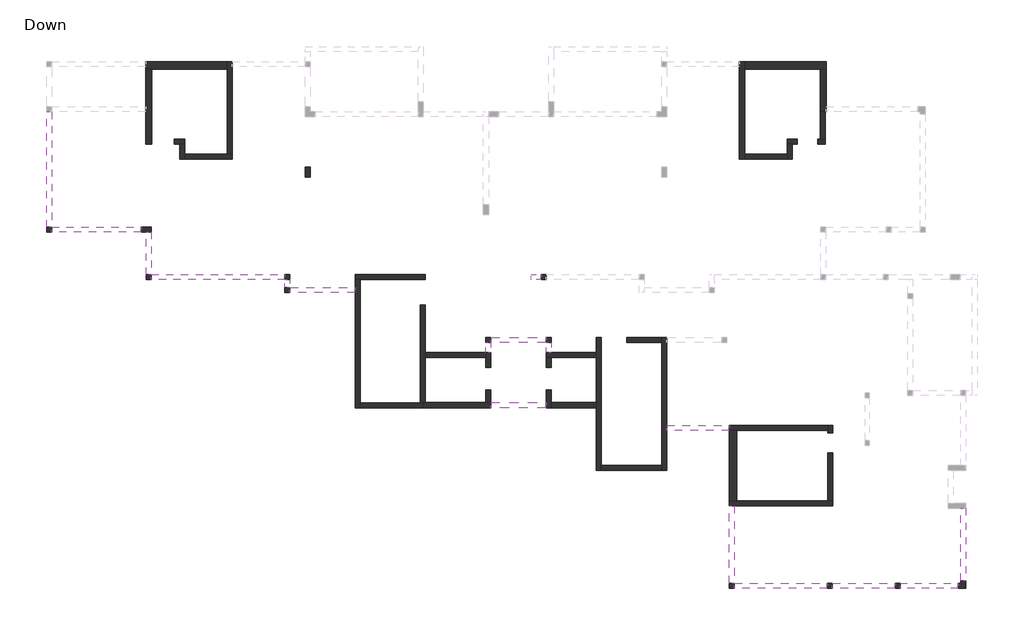
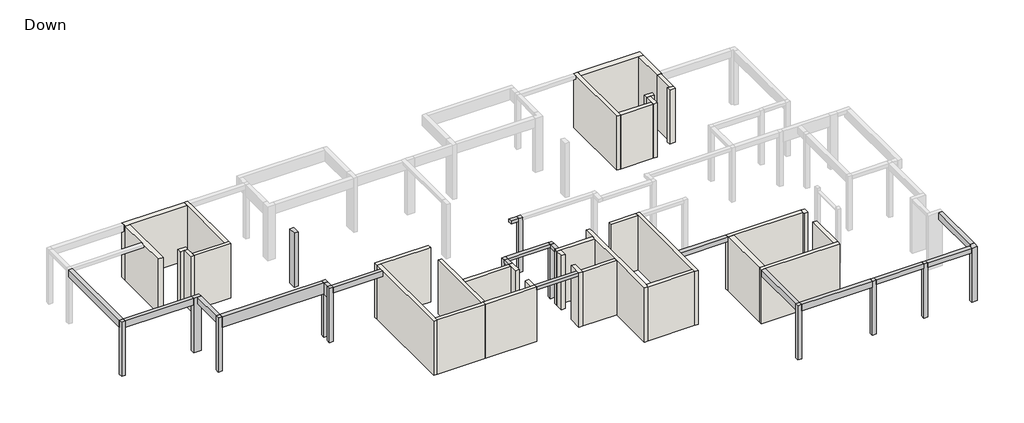
# One storey, part 1 of 2: 35 walls, 17 beams, 13 columns.
"""IFC4 building model written with IfcOpenShell, lengths in millimetres."""

from ifc_helpers import new_model, si_unit, frame, origin, origin_with_axes, place, context, project, spatial, polyline, outline, extrude, faceted_brep, element, save

model = new_model("IFC4")

# Units and contexts
model_context = context("Model", 3, world=origin())
ifc_project = project(units=[si_unit("LENGTHUNIT", "METRE", prefix="MILLI")], contexts=[model_context])

# Site, building, storey
site = spatial("IfcSite", under=ifc_project)
building = spatial("IfcBuilding", under=site)
storey = spatial("IfcBuildingStorey", under=building, Name="Down", Elevation=0.0)

# Beams
placement = place(None, origin())
element("IfcBeam", 1, ObjectType="Concrete Rectengular Beam : 20/15", at=placement, inside=storey, context=model_context, shape_type="SweptSolid", body=[
    extrude(outline(polyline([(23683.1266142, -26322.9713632), (23683.1266142, -26522.9713632), (21465.0782187, -26522.9713632), (21465.0782187, -26322.9713632), (23683.1266142, -26322.9713632)])), frame((0.0, 0.0, 2850.0), z_axis=(0.0, 0.0, 1.0), x_axis=(1.0, 0.0, 0.0)), (0.0, 0.0, 1.0), 150.0),
])
element("IfcBeam", 2, ObjectType="Concrete Rectengular Beam : 20/16", at=placement, inside=storey, context=model_context, shape_type="SweptSolid", body=[
    extrude(outline(polyline([(23683.1266142, -23722.9713632), (23683.1266142, -23922.9713632), (21465.0782187, -23922.9713632), (21465.0782187, -23722.9713632), (23683.1266142, -23722.9713632)])), frame((0.0, 0.0, 2840.0), z_axis=(0.0, 0.0, 1.0), x_axis=(1.0, 0.0, 0.0)), (0.0, 0.0, 1.0), 160.0),
])
element("IfcBeam", 3, ObjectType="Concrete Rectengular Beam : 20/16", at=placement, inside=storey, context=model_context, shape_type="SweptSolid", body=[
    extrude(outline(polyline([(23683.1266142, -23922.9713632), (23883.1266142, -23922.9713632), (23883.1266142, -24325.0312743), (23683.1266142, -24325.0312743), (23683.1266142, -23922.9713632)])), frame((0.0, 0.0, 2840.0), z_axis=(0.0, 0.0, 1.0), x_axis=(1.0, 0.0, 0.0)), (0.0, 0.0, 1.0), 160.0),
])
element("IfcBeam", 4, ObjectType="Concrete Rectengular Beam : 20/16", at=placement, inside=storey, context=model_context, shape_type="SweptSolid", body=[
    extrude(outline(polyline([(21265.0782187, -23922.9713632), (21465.0782187, -23922.9713632), (21465.0782187, -24325.0312743), (21265.0782187, -24325.0312743), (21265.0782187, -23922.9713632)])), frame((0.0, 0.0, 2840.0), z_axis=(0.0, 0.0, 1.0), x_axis=(1.0, 0.0, 0.0)), (0.0, 0.0, 1.0), 160.0),
])
element("IfcBeam", 5, ObjectType="Concrete Rectengular Beam : 20/16", at=placement, inside=storey, context=model_context, shape_type="Brep", body=[
    faceted_brep([(23078.0627315, -21217.3313694, 3000.0), (23078.0627315, -21217.3313694, 2840.0), (23078.0627315, -21325.0312743, 2840.0), (23078.0627315, -21417.3313694, 2840.0), (23078.0627315, -21417.3313694, 3000.0), (23078.0627315, -21325.0312743, 3000.0), (23478.0627315, -21417.3313694, 3000.0), (23478.0627315, -21217.3313694, 3000.0), (23478.0627315, -21217.3313694, 2840.0), (23478.0627315, -21417.3313694, 2840.0)], [[[0, 1, 2, 3, 4, 5]], [[4, 6, 7, 0, 5]], [[1, 0, 7, 8]], [[1, 8, 9, 3, 2]], [[4, 3, 9, 6]], [[7, 6, 9, 8]]]),
])
element("IfcBeam", 6, ObjectType="Concrete Rectengular Beam : 20/25", at=placement, inside=storey, context=model_context, shape_type="SweptSolid", body=[
    extrude(outline(polyline([(37784.3945148, -33727.8618321), (37784.3945148, -33527.8618321), (40096.0050664, -33527.8618321), (40096.0050664, -33727.8618321), (37784.3945148, -33727.8618321)])), frame((0.0, 0.0, 2750.0), z_axis=(0.0, 0.0, 1.0), x_axis=(1.0, 0.0, 0.0)), (0.0, 0.0, 1.0), 250.0),
])
element("IfcBeam", 7, ObjectType="Concrete Rectengular Beam : 20/25", at=placement, inside=storey, context=model_context, shape_type="SweptSolid", body=[
    extrude(outline(polyline([(35086.984967, -33727.8618321), (35086.984967, -33527.8618321), (37584.3945148, -33527.8618321), (37584.3945148, -33727.8618321), (35086.984967, -33727.8618321)])), frame((0.0, 0.0, 2750.0), z_axis=(0.0, 0.0, 1.0), x_axis=(1.0, 0.0, 0.0)), (0.0, 0.0, 1.0), 250.0),
])
element("IfcBeam", 8, ObjectType="Concrete Rectengular Beam : 20/25", at=placement, inside=storey, context=model_context, shape_type="Brep", body=[
    faceted_brep([(30975.7730306, -27429.5129889, 3000.0), (30975.7730306, -27229.5129889, 3000.0), (28484.6380738, -27229.5129889, 3000.0), (28484.6380738, -27429.5129889, 3000.0), (30975.7730306, -27229.5129889, 2840.0), (30975.7730306, -27229.5129889, 2750.0), (28484.6380738, -27229.5129889, 2750.0), (28484.6380738, -27229.5129889, 2840.0), (30975.7730306, -27429.5129889, 2750.0), (28484.6380738, -27429.5129889, 2750.0)], [[[0, 1, 2, 3]], [[2, 1, 4, 5, 6, 7]], [[5, 8, 9, 6]], [[8, 0, 3, 9]], [[1, 0, 8, 5, 4]], [[3, 2, 7, 6, 9]]]),
])
element("IfcBeam", 9, ObjectType="Concrete Rectengular Beam : 20/30", at=placement, inside=storey, context=model_context, shape_type="Brep", body=[
    faceted_brep([(13465.4456872, -21724.9991523, 3000.0), (13465.4456872, -21924.9991523, 3000.0), (16065.0782187, -21924.9991523, 3000.0), (16065.0782187, -21724.9991523, 3000.0), (13465.4456872, -21924.9991523, 2700.0), (16065.0782187, -21924.9991523, 2700.0), (13465.4456872, -21724.9991523, 2700.0), (16065.0782187, -21724.9991523, 2700.0), (16065.0782187, -21724.9991523, 2840.0), (13465.4456872, -21724.9991523, 2840.0)], [[[0, 1, 2, 3]], [[1, 4, 5, 2]], [[4, 6, 7, 5]], [[0, 3, 8, 7, 6, 9]], [[4, 1, 0, 9, 6]], [[3, 2, 5, 7, 8]]]),
])
element("IfcBeam", 10, ObjectType="Concrete Rectengular Beam : 20/35", at=placement, inside=storey, context=model_context, shape_type="Brep", body=[
    faceted_brep([(3964.5925114, -19324.5221497, 3000.0), (3964.5925114, -19524.5221497, 3000.0), (7532.8726521, -19524.5221497, 3000.0), (7532.8726521, -19324.5221497, 3000.0), (3964.5925114, -19524.5221497, 2650.0), (7532.8726521, -19524.5221497, 2650.0), (3964.5925114, -19324.5221497, 2650.0), (7532.8726521, -19324.5221497, 2650.0), (7532.8726521, -19324.5221497, 2840.0), (3964.5925114, -19324.5221497, 2840.0)], [[[0, 1, 2, 3]], [[1, 4, 5, 2]], [[4, 6, 7, 5]], [[0, 3, 8, 7, 6, 9]], [[4, 1, 0, 9, 6]], [[3, 2, 5, 7, 8]]]),
])
element("IfcBeam", 11, ObjectType="Concrete Rectengular Beam : 20/35", at=placement, inside=storey, context=model_context, shape_type="Brep", body=[
    faceted_brep([(7732.8726521, -21217.3313694, 3000.0), (7932.8726521, -21217.3313694, 3000.0), (7932.8726521, -19524.5221497, 3000.0), (7732.8726521, -19524.5221497, 3000.0), (7732.8726521, -21217.3313694, 2650.0), (7732.8726521, -19524.5221497, 2650.0), (7932.8726521, -21217.3313694, 2650.0), (7932.8726521, -19524.5221497, 2650.0), (7932.8726521, -21217.3313694, 2840.0), (7932.8726521, -19524.5221497, 2840.0)], [[[0, 1, 2, 3]], [[4, 0, 3, 5]], [[6, 4, 5, 7]], [[2, 1, 8, 6, 7, 9]], [[3, 2, 9, 7, 5]], [[1, 0, 4, 6, 8]]]),
])
element("IfcBeam", 12, ObjectType="Concrete Rectengular Beam : 20/35", at=placement, inside=storey, context=model_context, shape_type="Brep", body=[
    faceted_brep([(40196.0050664, -33427.8618321, 3000.0), (40396.0050664, -33427.8618321, 3000.0), (40396.0050664, -30530.1793317, 3000.0), (40196.0050664, -30530.1793317, 3000.0), (40196.0050664, -33427.8618321, 2650.0), (40196.0050664, -30530.1793317, 2840.0), (40196.0050664, -30530.1793317, 2650.0), (40396.0050664, -33427.8618321, 2650.0), (40396.0050664, -30530.1793317, 2650.0)], [[[0, 1, 2, 3]], [[4, 0, 3, 5, 6]], [[7, 4, 6, 8]], [[1, 7, 8, 2]], [[1, 0, 4, 7]], [[3, 2, 8, 6, 5]]]),
])
element("IfcBeam", 13, ObjectType="Concrete Rectengular Beam : 20/35", at=placement, inside=storey, context=model_context, shape_type="Brep", body=[
    faceted_brep([(31180.4949796, -33527.8618321, 3000.0), (31180.4949796, -33727.8618321, 3000.0), (34886.984967, -33727.8618321, 3000.0), (34886.984967, -33527.8618321, 3000.0), (31180.4949796, -33527.8618321, 2650.0), (31180.4949796, -33527.8618321, 2840.0), (34886.984967, -33527.8618321, 2650.0), (31180.4949796, -33727.8618321, 2650.0), (34886.984967, -33727.8618321, 2650.0)], [[[0, 1, 2, 3]], [[4, 5, 0, 3, 6]], [[7, 4, 6, 8]], [[1, 7, 8, 2]], [[1, 0, 5, 4, 7]], [[3, 2, 8, 6]]]),
])
element("IfcBeam", 14, ObjectType="Concrete Rectengular Beam : 20/35", at=placement, inside=storey, context=model_context, shape_type="Brep", body=[
    faceted_brep([(30980.4949796, -33527.8618321, 3000.0), (31180.4949796, -33527.8618321, 3000.0), (31180.4949796, -30429.5129889, 3000.0), (30980.4949796, -30429.5129889, 3000.0), (31180.4949796, -33527.8618321, 2840.0), (31180.4949796, -33527.8618321, 2650.0), (31180.4949796, -30429.5129889, 2650.0), (31180.4949796, -30429.5129889, 2840.0), (30980.4949796, -33527.8618321, 2650.0), (30980.4949796, -30429.5129889, 2650.0)], [[[0, 1, 2, 3]], [[1, 4, 5, 6, 7, 2]], [[5, 8, 9, 6]], [[8, 0, 3, 9]], [[0, 8, 5, 4, 1]], [[3, 2, 7, 6, 9]]]),
])
element("IfcBeam", 15, ObjectType="Concrete Rectengular Beam : 20/40", at=placement, inside=storey, context=model_context, shape_type="Brep", body=[
    faceted_brep([(3964.5925114, -14717.2626845, 3000.0), (3764.5925114, -14717.2626845, 3000.0), (3764.5925114, -19324.5221497, 3000.0), (3964.5925114, -19324.5221497, 3000.0), (3764.5925114, -14717.2626845, 2600.0), (3764.5925114, -19324.5221497, 2600.0), (3964.5925114, -14717.2626845, 2600.0), (3964.5925114, -19324.5221497, 2600.0), (3964.5925114, -14717.2626845, 2840.0), (3964.5925114, -19324.5221497, 2840.0)], [[[0, 1, 2, 3]], [[1, 4, 5, 2]], [[4, 6, 7, 5]], [[6, 8, 0, 3, 9, 7]], [[1, 0, 8, 6, 4]], [[3, 2, 5, 7, 9]]]),
])
element("IfcBeam", 16, ObjectType="Concrete Rectengular Beam : 20/60", at=placement, inside=storey, context=model_context, shape_type="Brep", body=[
    faceted_brep([(7932.8726521, -21217.3313694, 3000.0), (7932.8726521, -21417.3313694, 3000.0), (13265.4456872, -21417.3313694, 3000.0), (13265.4456872, -21217.3313694, 3000.0), (7932.8726521, -21417.3313694, 2400.0), (13265.4456872, -21417.3313694, 2400.0), (7932.8726521, -21217.3313694, 2400.0), (13265.4456872, -21217.3313694, 2400.0), (13265.4456872, -21217.3313694, 2840.0), (7932.8726521, -21217.3313694, 2840.0)], [[[0, 1, 2, 3]], [[1, 4, 5, 2]], [[4, 6, 7, 5]], [[0, 3, 8, 7, 6, 9]], [[1, 0, 9, 6, 4]], [[3, 2, 5, 7, 8]]]),
])
element("IfcBeam", 17, ObjectType="Concrete Rectengular Beam : 20/60", at=placement, inside=storey, context=model_context, shape_type="Brep", body=[
    faceted_brep([(13465.4456872, -21417.3313694, 3000.0), (13265.4456872, -21417.3313694, 3000.0), (13265.4456872, -21724.9991523, 3000.0), (13465.4456872, -21724.9991523, 3000.0), (13265.4456872, -21417.3313694, 2400.0), (13265.4456872, -21724.9991523, 2400.0), (13465.4456872, -21417.3313694, 2400.0), (13465.4456872, -21724.9991523, 2400.0), (13465.4456872, -21724.9991523, 2840.0), (13465.4456872, -21417.3313694, 2840.0)], [[[0, 1, 2, 3]], [[1, 4, 5, 2]], [[4, 6, 7, 5]], [[0, 3, 8, 7, 6, 9]], [[4, 1, 0, 9, 6]], [[3, 2, 5, 7, 8]]]),
])

# Columns
element("IfcColumn", 18, ObjectType="Concrete Rectengular Column : 20/20", at=placement, inside=storey, context=model_context, shape_type="SweptSolid", body=[
    extrude(outline(polyline([(31180.4949796, -33527.8618321), (31180.4949796, -33727.8618321), (30980.4949796, -33727.8618321), (30980.4949796, -33527.8618321), (31180.4949796, -33527.8618321)])), origin_with_axes(), (0.0, 0.0, 1.0), 3000.0),
])
element("IfcColumn", 19, ObjectType="Concrete Rectengular Column : 20/20", at=placement, inside=storey, context=model_context, shape_type="SweptSolid", body=[
    extrude(outline(polyline([(35086.984967, -33527.8618321), (35086.984967, -33727.8618321), (34886.984967, -33727.8618321), (34886.984967, -33527.8618321), (35086.984967, -33527.8618321)])), origin_with_axes(), (0.0, 0.0, 1.0), 3000.0),
])
element("IfcColumn", 20, ObjectType="Concrete Rectengular Column : 20/20", at=placement, inside=storey, context=model_context, shape_type="SweptSolid", body=[
    extrude(outline(polyline([(37784.3945148, -33527.8618321), (37784.3945148, -33727.8618321), (37584.3945148, -33727.8618321), (37584.3945148, -33527.8618321), (37784.3945148, -33527.8618321)])), origin_with_axes(), (0.0, 0.0, 1.0), 3000.0),
])
element("IfcColumn", 21, ObjectType="Concrete Rectengular Column : 20/20", at=placement, inside=storey, context=model_context, shape_type="SweptSolid", body=[
    extrude(outline(polyline([(23678.0627315, -21217.3313694), (23678.0627315, -21417.3313694), (23478.0627315, -21417.3313694), (23478.0627315, -21217.3313694), (23678.0627315, -21217.3313694)])), origin_with_axes(), (0.0, 0.0, 1.0), 3000.0),
])
element("IfcColumn", 22, ObjectType="Concrete Rectengular Column : 20/20", at=placement, inside=storey, context=model_context, shape_type="Brep", body=[
    faceted_brep([(23883.1266142, -23722.9713632, 0.0), (23883.1266142, -23922.9713632, 0.0), (23683.1266142, -23922.9713632, 0.0), (23683.1266142, -23722.9713632, 0.0), (23883.1266142, -23722.9713632, 3000.0), (23883.1266142, -23922.9713632, 3000.0), (23883.1266142, -23722.9713632, 2840.0), (23683.1266142, -23922.9713632, 3000.0), (23683.1266142, -23722.9713632, 3000.0)], [[[0, 1, 2, 3]], [[4, 5, 1, 0, 6]], [[5, 7, 2, 1]], [[7, 8, 3, 2]], [[8, 4, 6, 0, 3]], [[4, 8, 7, 5]]]),
])
element("IfcColumn", 23, ObjectType="Concrete Rectengular Column : 20/20", at=placement, inside=storey, context=model_context, shape_type="Brep", body=[
    faceted_brep([(21465.0782187, -23722.9713632, 0.0), (21465.0782187, -23922.9713632, 0.0), (21265.0782187, -23922.9713632, 0.0), (21265.0782187, -23722.9713632, 0.0), (21465.0782187, -23722.9713632, 3000.0), (21465.0782187, -23922.9713632, 3000.0), (21265.0782187, -23922.9713632, 3000.0), (21265.0782187, -23722.9713632, 3000.0), (21265.0782187, -23722.9713632, 2840.0)], [[[0, 1, 2, 3]], [[4, 5, 1, 0]], [[5, 6, 2, 1]], [[6, 7, 8, 3, 2]], [[7, 4, 0, 3, 8]], [[4, 7, 6, 5]]]),
])
element("IfcColumn", 24, ObjectType="Concrete Rectengular Column : 20/20", at=placement, inside=storey, context=model_context, shape_type="SweptSolid", body=[
    extrude(outline(polyline([(3964.5925114, -19324.5221497), (3964.5925114, -19524.5221497), (3764.5925114, -19524.5221497), (3764.5925114, -19324.5221497), (3964.5925114, -19324.5221497)])), origin_with_axes(), (0.0, 0.0, 1.0), 3000.0),
])
element("IfcColumn", 25, ObjectType="Concrete Rectengular Column : 20/20", at=placement, inside=storey, context=model_context, shape_type="SweptSolid", body=[
    extrude(outline(polyline([(7932.8726521, -21217.3313694), (7932.8726521, -21417.3313694), (7732.8726521, -21417.3313694), (7732.8726521, -21217.3313694), (7932.8726521, -21217.3313694)])), origin_with_axes(), (0.0, 0.0, 1.0), 3000.0),
])
element("IfcColumn", 26, ObjectType="Concrete Rectengular Column : 20/20", at=placement, inside=storey, context=model_context, shape_type="Brep", body=[
    faceted_brep([(13465.4456872, -21217.3313694, 0.0), (13465.4456872, -21417.3313694, 0.0), (13265.4456872, -21417.3313694, 0.0), (13265.4456872, -21217.3313694, 0.0), (13465.4456872, -21217.3313694, 3000.0), (13465.4456872, -21417.3313694, 3000.0), (13465.4456872, -21217.3313694, 2840.0), (13265.4456872, -21417.3313694, 3000.0), (13265.4456872, -21217.3313694, 3000.0)], [[[0, 1, 2, 3]], [[4, 5, 1, 0, 6]], [[5, 7, 2, 1]], [[7, 8, 3, 2]], [[8, 4, 6, 0, 3]], [[4, 8, 7, 5]]]),
])
element("IfcColumn", 27, ObjectType="Concrete Rectengular Column : 20/20", at=placement, inside=storey, context=model_context, shape_type="SweptSolid", body=[
    extrude(outline(polyline([(13465.4456872, -21724.9991523), (13465.4456872, -21924.9991523), (13265.4456872, -21924.9991523), (13265.4456872, -21724.9991523), (13465.4456872, -21724.9991523)])), origin_with_axes(), (0.0, 0.0, 1.0), 3000.0),
])
element("IfcColumn", 28, ObjectType="Concrete Rectengular Column : 20/40", at=placement, inside=storey, context=model_context, shape_type="Brep", body=[
    faceted_brep([(7532.8726521, -19324.5221497, 0.0), (7932.8726521, -19324.5221497, 0.0), (7932.8726521, -19524.5221497, 0.0), (7532.8726521, -19524.5221497, 0.0), (7532.8726521, -19324.5221497, 3000.0), (7932.8726521, -19324.5221497, 3000.0), (7932.8726521, -19324.5221497, 2840.0), (7932.8726521, -19524.5221497, 3000.0), (7532.8726521, -19524.5221497, 3000.0)], [[[0, 1, 2, 3]], [[4, 5, 6, 1, 0]], [[5, 7, 2, 1, 6]], [[7, 8, 3, 2]], [[8, 4, 0, 3]], [[4, 8, 7, 5]]]),
])
element("IfcColumn", 29, ObjectType="Concrete Rectengular Column : 20/40", at=placement, inside=storey, context=model_context, shape_type="Brep", body=[
    faceted_brep([(14276.6245949, -16922.7697624, 0.0), (14276.6245949, -17322.7697624, 0.0), (14076.6245949, -17322.7697624, 0.0), (14076.6245949, -16922.7697624, 0.0), (14276.6245949, -16922.7697624, 3000.0), (14276.6245949, -17322.7697624, 3000.0), (14276.6245949, -17322.7697624, 2840.0), (14276.6245949, -16922.7697624, 2840.0), (14076.6245949, -17322.7697624, 3000.0), (14076.6245949, -17322.7697624, 2840.0), (14076.6245949, -16922.7697624, 3000.0), (14076.6245949, -16922.7697624, 2840.0)], [[[0, 1, 2, 3]], [[4, 5, 6, 1, 0, 7]], [[5, 8, 9, 2, 1, 6]], [[8, 10, 11, 3, 2, 9]], [[10, 4, 7, 0, 3, 11]], [[4, 10, 8, 5]]]),
])
element("IfcColumn", 30, ObjectType="L Column : 30/30/20/20", at=placement, inside=storey, context=model_context, shape_type="Brep", body=[
    faceted_brep([(40396.0050664, -33727.8618321, 0.0), (40096.0050664, -33727.8618321, 0.0), (40096.0050664, -33527.8618321, 0.0), (40196.0050664, -33527.8618321, 0.0), (40196.0050664, -33427.8618321, 0.0), (40396.0050664, -33427.8618321, 0.0), (40396.0050664, -33727.8618321, 3000.0), (40096.0050664, -33727.8618321, 3000.0), (40096.0050664, -33527.8618321, 3000.0), (40196.0050664, -33527.8618321, 3000.0), (40196.0050664, -33527.8618321, 2840.0), (40196.0050664, -33427.8618321, 3000.0), (40396.0050664, -33427.8618321, 3000.0)], [[[0, 1, 2, 3, 4, 5]], [[6, 7, 1, 0]], [[7, 8, 2, 1]], [[8, 9, 10, 3, 2]], [[9, 11, 4, 3, 10]], [[11, 12, 5, 4]], [[12, 6, 0, 5]], [[6, 12, 11, 9, 8, 7]]]),
])

# Walls
element("IfcWall", 31, ObjectType="20", at=placement, inside=storey, context=model_context, shape_type="Brep", body=[
    faceted_brep([(8856.7769333, -16016.1045626, 0.0), (9066.7769333, -16016.1045626, 0.0), (9266.7769333, -16016.1045626, 0.0), (9266.7769333, -16016.1045626, 3000.0), (9066.7769333, -16016.1045626, 3000.0), (8856.7769333, -16016.1045626, 3000.0), (8856.7769333, -16016.1045626, 2840.0), (8856.7769333, -15816.1045626, 0.0), (8856.7769333, -15816.1045626, 2840.0), (8856.7769333, -15816.1045626, 3000.0), (9266.7769333, -15816.1045626, 3000.0), (9266.7769333, -15816.1045626, 2840.0), (9266.7769333, -15816.1045626, 0.0)], [[[0, 1, 2, 3, 4, 5, 6]], [[7, 8, 9, 10, 11, 12]], [[2, 1, 0, 7, 12]], [[5, 4, 3, 10, 9]], [[0, 6, 5, 9, 8, 7]], [[3, 2, 12, 11, 10]]]),
])
element("IfcWall", 32, ObjectType="20", at=placement, inside=storey, context=model_context, shape_type="Brep", body=[
    faceted_brep([(9066.7769333, -16016.1045626, 0.0), (9066.7769333, -16605.3286465, 0.0), (9066.7769333, -16605.3286465, 2840.0), (9066.7769333, -16605.3286465, 3000.0), (9066.7769333, -16016.1045626, 3000.0), (9066.7769333, -16016.1045626, 2840.0), (9266.7769333, -16016.1045626, 0.0), (9266.7769333, -16016.1045626, 3000.0), (9266.7769333, -16405.3286465, 3000.0), (9266.7769333, -16605.3286465, 3000.0), (9266.7769333, -16605.3286465, 0.0), (9266.7769333, -16405.3286465, 0.0)], [[[0, 1, 2, 3, 4, 5]], [[6, 7, 8, 9, 10, 11]], [[1, 0, 6, 11, 10]], [[4, 3, 9, 8, 7]], [[0, 5, 4, 7, 6]], [[3, 2, 1, 10, 9]]]),
])
element("IfcWall", 33, ObjectType="20", at=placement, inside=storey, context=model_context, shape_type="Brep", body=[
    faceted_brep([(9266.7769333, -16605.3286465, 0.0), (11166.7769333, -16605.3286465, 0.0), (11166.7769333, -16605.3286465, 2840.0), (11166.7769333, -16605.3286465, 3000.0), (9266.7769333, -16605.3286465, 3000.0), (9266.7769333, -16405.3286465, 0.0), (9266.7769333, -16405.3286465, 2840.0), (9266.7769333, -16405.3286465, 3000.0), (10966.7769333, -16405.3286465, 3000.0), (11166.7769333, -16405.3286465, 3000.0), (11166.7769333, -16405.3286465, 0.0), (10966.7769333, -16405.3286465, 0.0)], [[[0, 1, 2, 3, 4]], [[5, 6, 7, 8, 9, 10, 11]], [[1, 0, 5, 11, 10]], [[4, 3, 9, 8, 7]], [[0, 4, 7, 6, 5]], [[3, 2, 1, 10, 9]]]),
])
element("IfcWall", 34, ObjectType="20", at=placement, inside=storey, context=model_context, shape_type="Brep", body=[
    faceted_brep([(11166.7769333, -16405.3286465, 0.0), (11166.7769333, -12716.1045626, 0.0), (11166.7769333, -12716.1045626, 3000.0), (11166.7769333, -12916.1045626, 3000.0), (11166.7769333, -16405.3286465, 3000.0), (10966.7769333, -16405.3286465, 0.0), (10966.7769333, -16405.3286465, 2840.0), (10966.7769333, -16405.3286465, 3000.0), (10966.7769333, -13016.1045626, 3000.0), (10966.7769333, -12716.1045626, 3000.0), (10966.7769333, -12716.1045626, 0.0), (10966.7769333, -13016.1045626, 0.0)], [[[0, 1, 2, 3, 4]], [[5, 6, 7, 8, 9, 10, 11]], [[1, 0, 5, 11, 10]], [[4, 3, 2, 9, 8, 7]], [[0, 4, 7, 6, 5]], [[2, 1, 10, 9]]]),
])
element("IfcWall", 35, ObjectType="20", at=placement, inside=storey, context=model_context, shape_type="Brep", body=[
    faceted_brep([(35091.7617084, -30229.5129889, 0.0), (34891.7617084, -30229.5129889, 0.0), (31275.7730306, -30229.5129889, 0.0), (30975.7730306, -30229.5129889, 0.0), (30975.7730306, -30229.5129889, 3000.0), (31275.7730306, -30229.5129889, 3000.0), (34891.7617084, -30229.5129889, 3000.0), (35091.7617084, -30229.5129889, 3000.0), (35091.7617084, -30429.5129889, 0.0), (35091.7617084, -30429.5129889, 2840.0), (35091.7617084, -30429.5129889, 3000.0), (31180.4949796, -30429.5129889, 3000.0), (30980.4949796, -30429.5129889, 3000.0), (30975.7730306, -30429.5129889, 3000.0), (30975.7730306, -30429.5129889, 0.0)], [[[0, 1, 2, 3, 4, 5, 6, 7]], [[8, 9, 10, 11, 12, 13, 14]], [[3, 2, 1, 0, 8, 14]], [[7, 6, 5, 4, 13, 12, 11, 10]], [[0, 7, 10, 9, 8]], [[4, 3, 14, 13]]]),
])
element("IfcWall", 36, ObjectType="20", at=placement, inside=storey, context=model_context, shape_type="Brep", body=[
    faceted_brep([(35091.7617084, -30229.5129889, 0.0), (35091.7617084, -28329.5129889, 0.0), (35091.7617084, -28329.5129889, 2840.0), (35091.7617084, -28329.5129889, 3000.0), (35091.7617084, -30229.5129889, 3000.0), (34891.7617084, -30229.5129889, 0.0), (34891.7617084, -30229.5129889, 2840.0), (34891.7617084, -30229.5129889, 3000.0), (34891.7617084, -28329.5129889, 3000.0), (34891.7617084, -28329.5129889, 2840.0), (34891.7617084, -28329.5129889, 0.0)], [[[0, 1, 2, 3, 4]], [[5, 6, 7, 8, 9, 10]], [[1, 0, 5, 10]], [[3, 2, 1, 10, 9, 8]], [[4, 3, 8, 7]], [[0, 4, 7, 6, 5]]]),
])
element("IfcWall", 37, ObjectType="20", at=placement, inside=storey, context=model_context, shape_type="Brep", body=[
    faceted_brep([(35091.7617084, -27529.5129889, 0.0), (35091.7617084, -27229.5129889, 0.0), (35091.7617084, -27229.5129889, 2840.0), (35091.7617084, -27229.5129889, 3000.0), (35091.7617084, -27529.5129889, 3000.0), (35091.7617084, -27529.5129889, 2840.0), (34891.7617084, -27529.5129889, 0.0), (34891.7617084, -27529.5129889, 2840.0), (34891.7617084, -27529.5129889, 3000.0), (34891.7617084, -27429.5129889, 3000.0), (34891.7617084, -27229.5129889, 3000.0), (34891.7617084, -27229.5129889, 0.0), (34891.7617084, -27429.5129889, 0.0)], [[[0, 1, 2, 3, 4, 5]], [[6, 7, 8, 9, 10, 11, 12]], [[1, 0, 6, 12, 11]], [[4, 3, 10, 9, 8]], [[0, 5, 4, 8, 7, 6]], [[3, 2, 1, 11, 10]]]),
])
element("IfcWall", 38, ObjectType="20", at=placement, inside=storey, context=model_context, shape_type="Brep", body=[
    faceted_brep([(34891.7617084, -27229.5129889, 0.0), (30975.7730306, -27229.5129889, 0.0), (30975.7730306, -27229.5129889, 2750.0), (30975.7730306, -27229.5129889, 3000.0), (34891.7617084, -27229.5129889, 3000.0), (34891.7617084, -27429.5129889, 0.0), (34891.7617084, -27429.5129889, 2840.0), (34891.7617084, -27429.5129889, 3000.0), (31275.7730306, -27429.5129889, 3000.0), (30975.7730306, -27429.5129889, 3000.0), (30975.7730306, -27429.5129889, 2750.0), (30975.7730306, -27429.5129889, 0.0), (31275.7730306, -27429.5129889, 0.0)], [[[0, 1, 2, 3, 4]], [[5, 6, 7, 8, 9, 10, 11, 12]], [[1, 0, 5, 12, 11]], [[4, 3, 9, 8, 7]], [[0, 4, 7, 6, 5]], [[3, 2, 1, 11, 10, 9]]]),
])
element("IfcWall", 39, ObjectType="20", at=placement, inside=storey, context=model_context, shape_type="Brep", body=[
    faceted_brep([(28484.6380738, -29030.0312743, 0.0), (28484.6380738, -23722.9713632, 0.0), (28484.6380738, -23722.9713632, 3000.0), (28484.6380738, -23922.9713632, 3000.0), (28484.6380738, -27229.5129889, 3000.0), (28484.6380738, -29030.0312743, 3000.0), (28284.6380738, -29030.0312743, 0.0), (28284.6380738, -29030.0312743, 3000.0), (28284.6380738, -28830.0312743, 3000.0), (28284.6380738, -23922.9713632, 3000.0), (28284.6380738, -23722.9713632, 3000.0), (28284.6380738, -23722.9713632, 0.0), (28284.6380738, -23922.9713632, 0.0), (28284.6380738, -28830.0312743, 0.0)], [[[0, 1, 2, 3, 4, 5]], [[6, 7, 8, 9, 10, 11, 12, 13]], [[1, 0, 6, 13, 12, 11]], [[5, 4, 3, 2, 10, 9, 8, 7]], [[2, 1, 11, 10]], [[0, 5, 7, 6]]]),
])
element("IfcWall", 40, ObjectType="20", at=placement, inside=storey, context=model_context, shape_type="Brep", body=[
    faceted_brep([(28284.6380738, -23722.9713632, 0.0), (26884.6380738, -23722.9713632, 0.0), (26884.6380738, -23722.9713632, 2840.0), (26884.6380738, -23722.9713632, 3000.0), (28284.6380738, -23722.9713632, 3000.0), (28284.6380738, -23922.9713632, 0.0), (28284.6380738, -23922.9713632, 3000.0), (26884.6380738, -23922.9713632, 3000.0), (26884.6380738, -23922.9713632, 2840.0), (26884.6380738, -23922.9713632, 0.0)], [[[0, 1, 2, 3, 4]], [[5, 6, 7, 8, 9]], [[1, 0, 5, 9]], [[3, 2, 1, 9, 8, 7]], [[4, 3, 7, 6]], [[0, 4, 6, 5]]]),
])
element("IfcWall", 41, ObjectType="20", at=placement, inside=storey, context=model_context, shape_type="Brep", body=[
    faceted_brep([(25666.8915333, -23725.0312743, 0.0), (25666.8915333, -24325.0312743, 0.0), (25666.8915333, -24525.0312743, 0.0), (25666.8915333, -26322.9713632, 0.0), (25666.8915333, -26522.9713632, 0.0), (25666.8915333, -29030.0312743, 0.0), (25666.8915333, -29030.0312743, 3000.0), (25666.8915333, -26522.9713632, 3000.0), (25666.8915333, -26322.9713632, 3000.0), (25666.8915333, -24525.0312743, 3000.0), (25666.8915333, -24325.0312743, 3000.0), (25666.8915333, -23725.0312743, 3000.0), (25666.8915333, -23725.0312743, 2840.0), (25866.8915333, -23725.0312743, 0.0), (25866.8915333, -23725.0312743, 2840.0), (25866.8915333, -23725.0312743, 3000.0), (25866.8915333, -23922.9713632, 3000.0), (25866.8915333, -28830.0312743, 3000.0), (25866.8915333, -29030.0312743, 3000.0), (25866.8915333, -29030.0312743, 0.0), (25866.8915333, -28830.0312743, 0.0)], [[[0, 1, 2, 3, 4, 5, 6, 7, 8, 9, 10, 11, 12]], [[13, 14, 15, 16, 17, 18, 19, 20]], [[5, 4, 3, 2, 1, 0, 13, 20, 19]], [[11, 10, 9, 8, 7, 6, 18, 17, 16, 15]], [[0, 12, 11, 15, 14, 13]], [[6, 5, 19, 18]]]),
])
element("IfcWall", 42, ObjectType="20", at=placement, inside=storey, context=model_context, shape_type="SweptSolid", body=[
    extrude(outline(polyline([(28284.6380738, -29030.0312743), (25866.8915333, -29030.0312743), (25866.8915333, -28830.0312743), (28284.6380738, -28830.0312743), (28284.6380738, -29030.0312743)])), origin_with_axes(), (0.0, 0.0, 1.0), 3000.0),
])
element("IfcWall", 43, ObjectType="20", at=placement, inside=storey, context=model_context, shape_type="Brep", body=[
    faceted_brep([(25666.8915333, -24325.0312743, 0.0), (23683.1266142, -24325.0312743, 0.0), (23683.1266142, -24325.0312743, 3000.0), (23883.1266142, -24325.0312743, 3000.0), (25666.8915333, -24325.0312743, 3000.0), (25666.8915333, -24325.0312743, 2840.0), (25666.8915333, -24525.0312743, 0.0), (25666.8915333, -24525.0312743, 3000.0), (23883.1266142, -24525.0312743, 3000.0), (23683.1266142, -24525.0312743, 3000.0), (23683.1266142, -24525.0312743, 0.0), (23883.1266142, -24525.0312743, 0.0)], [[[0, 1, 2, 3, 4, 5]], [[6, 7, 8, 9, 10, 11]], [[1, 0, 6, 11, 10]], [[4, 3, 2, 9, 8, 7]], [[0, 5, 4, 7, 6]], [[2, 1, 10, 9]]]),
])
element("IfcWall", 44, ObjectType="20", at=placement, inside=storey, context=model_context, shape_type="Brep", body=[
    faceted_brep([(23683.1266142, -24525.0312743, 0.0), (23683.1266142, -24925.0312743, 0.0), (23683.1266142, -24925.0312743, 2840.0), (23683.1266142, -24925.0312743, 3000.0), (23683.1266142, -24525.0312743, 3000.0), (23883.1266142, -24525.0312743, 0.0), (23883.1266142, -24525.0312743, 3000.0), (23883.1266142, -24925.0312743, 3000.0), (23883.1266142, -24925.0312743, 2840.0), (23883.1266142, -24925.0312743, 0.0)], [[[0, 1, 2, 3, 4]], [[5, 6, 7, 8, 9]], [[1, 0, 5, 9]], [[3, 2, 1, 9, 8, 7]], [[4, 3, 7, 6]], [[0, 4, 6, 5]]]),
])
element("IfcWall", 45, ObjectType="20", at=placement, inside=storey, context=model_context, shape_type="Brep", body=[
    faceted_brep([(23683.1266142, -25822.9713632, 0.0), (23683.1266142, -26522.9713632, 0.0), (23683.1266142, -26522.9713632, 3000.0), (23683.1266142, -26322.9713632, 3000.0), (23683.1266142, -25822.9713632, 3000.0), (23683.1266142, -25822.9713632, 2840.0), (23883.1266142, -25822.9713632, 0.0), (23883.1266142, -25822.9713632, 2840.0), (23883.1266142, -25822.9713632, 3000.0), (23883.1266142, -26322.9713632, 3000.0), (23883.1266142, -26522.9713632, 3000.0), (23883.1266142, -26522.9713632, 0.0), (23883.1266142, -26322.9713632, 0.0)], [[[0, 1, 2, 3, 4, 5]], [[6, 7, 8, 9, 10, 11, 12]], [[1, 0, 6, 12, 11]], [[4, 3, 2, 10, 9, 8]], [[0, 5, 4, 8, 7, 6]], [[2, 1, 11, 10]]]),
])
element("IfcWall", 46, ObjectType="20", at=placement, inside=storey, context=model_context, shape_type="SweptSolid", body=[
    extrude(outline(polyline([(25666.8915333, -26522.9713632), (23883.1266142, -26522.9713632), (23883.1266142, -26322.9713632), (25666.8915333, -26322.9713632), (25666.8915333, -26522.9713632)])), origin_with_axes(), (0.0, 0.0, 1.0), 3000.0),
])
element("IfcWall", 47, ObjectType="20", at=placement, inside=storey, context=model_context, shape_type="Brep", body=[
    faceted_brep([(21465.0782187, -24925.0312743, 0.0), (21465.0782187, -24325.0312743, 0.0), (21465.0782187, -24325.0312743, 2840.0), (21465.0782187, -24325.0312743, 3000.0), (21465.0782187, -24925.0312743, 3000.0), (21465.0782187, -24925.0312743, 2840.0), (21265.0782187, -24925.0312743, 0.0), (21265.0782187, -24925.0312743, 2840.0), (21265.0782187, -24925.0312743, 3000.0), (21265.0782187, -24525.0312743, 3000.0), (21265.0782187, -24325.0312743, 3000.0), (21265.0782187, -24325.0312743, 2840.0), (21265.0782187, -24325.0312743, 0.0), (21265.0782187, -24525.0312743, 0.0)], [[[0, 1, 2, 3, 4, 5]], [[6, 7, 8, 9, 10, 11, 12, 13]], [[1, 0, 6, 13, 12]], [[4, 3, 10, 9, 8]], [[0, 5, 4, 8, 7, 6]], [[3, 2, 1, 12, 11, 10]]]),
])
element("IfcWall", 48, ObjectType="20", at=placement, inside=storey, context=model_context, shape_type="Brep", body=[
    faceted_brep([(21265.0782187, -24325.0312743, 0.0), (18865.0782187, -24325.0312743, 0.0), (18865.0782187, -24325.0312743, 2840.0), (18865.0782187, -24325.0312743, 3000.0), (21265.0782187, -24325.0312743, 3000.0), (21265.0782187, -24325.0312743, 2840.0), (21265.0782187, -24525.0312743, 0.0), (21265.0782187, -24525.0312743, 3000.0), (18865.0782187, -24525.0312743, 3000.0), (18865.0782187, -24525.0312743, 0.0)], [[[0, 1, 2, 3, 4, 5]], [[6, 7, 8, 9]], [[1, 0, 6, 9]], [[4, 3, 8, 7]], [[0, 5, 4, 7, 6]], [[3, 2, 1, 9, 8]]]),
])
element("IfcWall", 49, ObjectType="20", at=placement, inside=storey, context=model_context, shape_type="Brep", body=[
    faceted_brep([(18765.0782187, -26522.9713632, 0.0), (21465.0782187, -26522.9713632, 0.0), (21465.0782187, -26522.9713632, 2850.0), (21465.0782187, -26522.9713632, 3000.0), (18765.0782187, -26522.9713632, 3000.0), (18765.0782187, -26322.9713632, 0.0), (18765.0782187, -26322.9713632, 3000.0), (18865.0782187, -26322.9713632, 3000.0), (21265.0782187, -26322.9713632, 3000.0), (21465.0782187, -26322.9713632, 3000.0), (21465.0782187, -26322.9713632, 2850.0), (21465.0782187, -26322.9713632, 0.0), (21265.0782187, -26322.9713632, 0.0), (18865.0782187, -26322.9713632, 0.0), (18765.0782187, -26324.9991523, 0.0), (18765.0782187, -26324.9991523, 3000.0)], [[[0, 1, 2, 3, 4]], [[5, 6, 7, 8, 9, 10, 11, 12, 13]], [[1, 0, 14, 5, 13, 12, 11]], [[4, 3, 9, 8, 7, 6, 15]], [[0, 4, 15, 6, 5, 14]], [[3, 2, 1, 11, 10, 9]]]),
])
element("IfcWall", 50, ObjectType="20", at=placement, inside=storey, context=model_context, shape_type="Brep", body=[
    faceted_brep([(21465.0782187, -26322.9713632, 0.0), (21465.0782187, -25822.9713632, 0.0), (21465.0782187, -25822.9713632, 2840.0), (21465.0782187, -25822.9713632, 3000.0), (21465.0782187, -26322.9713632, 3000.0), (21465.0782187, -26322.9713632, 2840.0), (21265.0782187, -26322.9713632, 0.0), (21265.0782187, -26322.9713632, 3000.0), (21265.0782187, -25822.9713632, 3000.0), (21265.0782187, -25822.9713632, 2840.0), (21265.0782187, -25822.9713632, 0.0)], [[[0, 1, 2, 3, 4, 5]], [[6, 7, 8, 9, 10]], [[1, 0, 6, 10]], [[3, 2, 1, 10, 9, 8]], [[4, 3, 8, 7]], [[0, 5, 4, 7, 6]]]),
])
element("IfcWall", 51, ObjectType="20", at=placement, inside=storey, context=model_context, shape_type="Brep", body=[
    faceted_brep([(18865.0782187, -26322.9713632, 0.0), (18865.0782187, -24525.0312743, 0.0), (18865.0782187, -24325.0312743, 0.0), (18865.0782187, -22425.0312743, 0.0), (18865.0782187, -22425.0312743, 2840.0), (18865.0782187, -22425.0312743, 3000.0), (18865.0782187, -24325.0312743, 3000.0), (18865.0782187, -24525.0312743, 3000.0), (18865.0782187, -26322.9713632, 3000.0), (18665.0782187, -26324.9991523, 0.0), (18665.0782187, -26324.9991523, 3000.0), (18665.0782187, -22425.0312743, 3000.0), (18665.0782187, -22425.0312743, 2840.0), (18665.0782187, -22425.0312743, 0.0), (18765.0782187, -26322.9713632, 0.0), (18765.0782187, -26324.9991523, 0.0), (18765.0782187, -26324.9991523, 3000.0), (18765.0782187, -26322.9713632, 3000.0)], [[[0, 1, 2, 3, 4, 5, 6, 7, 8]], [[9, 10, 11, 12, 13]], [[3, 2, 1, 0, 14, 15, 9, 13]], [[5, 4, 3, 13, 12, 11]], [[8, 7, 6, 5, 11, 10, 16, 17]], [[0, 8, 17, 14]], [[17, 16, 15, 14]], [[16, 10, 9, 15]]]),
])
element("IfcWall", 52, ObjectType="20", at=placement, inside=storey, context=model_context, shape_type="Brep", body=[
    faceted_brep([(18865.0782187, -21204.9991523, 0.0), (16065.0782187, -21204.9991523, 0.0), (16065.0782187, -21204.9991523, 2840.0), (16065.0782187, -21204.9991523, 3000.0), (18865.0782187, -21204.9991523, 3000.0), (18865.0782187, -21204.9991523, 2840.0), (18865.0782187, -21404.9991523, 0.0), (18865.0782187, -21404.9991523, 2840.0), (18865.0782187, -21404.9991523, 3000.0), (18665.0782187, -21404.9991523, 3000.0), (16265.0782187, -21404.9991523, 3000.0), (16065.0782187, -21404.9991523, 3000.0), (16065.0782187, -21404.9991523, 0.0), (16265.0782187, -21404.9991523, 0.0)], [[[0, 1, 2, 3, 4, 5]], [[6, 7, 8, 9, 10, 11, 12, 13]], [[1, 0, 6, 13, 12]], [[4, 3, 11, 10, 9, 8]], [[0, 5, 4, 8, 7, 6]], [[3, 2, 1, 12, 11]]]),
])
element("IfcWall", 53, ObjectType="20", at=placement, inside=storey, context=model_context, shape_type="Brep", body=[
    faceted_brep([(16065.0782187, -21404.9991523, 0.0), (16065.0782187, -26524.9991523, 0.0), (16065.0782187, -26524.9991523, 3000.0), (16065.0782187, -21724.9991523, 3000.0), (16065.0782187, -21404.9991523, 3000.0), (16265.0782187, -21404.9991523, 0.0), (16265.0782187, -21404.9991523, 3000.0), (16265.0782187, -26324.9991523, 3000.0), (16265.0782187, -26524.9991523, 3000.0), (16265.0782187, -26524.9991523, 0.0), (16265.0782187, -26324.9991523, 0.0)], [[[0, 1, 2, 3, 4]], [[5, 6, 7, 8, 9, 10]], [[1, 0, 5, 10, 9]], [[4, 3, 2, 8, 7, 6]], [[0, 4, 6, 5]], [[2, 1, 9, 8]]]),
])
element("IfcWall", 54, ObjectType="20", at=placement, inside=storey, context=model_context, shape_type="Brep", body=[
    faceted_brep([(16265.0782187, -26524.9991523, 0.0), (18765.0782187, -26524.9991523, 0.0), (18765.0782187, -26524.9991523, 3000.0), (16265.0782187, -26524.9991523, 3000.0), (16265.0782187, -26324.9991523, 0.0), (16265.0782187, -26324.9991523, 3000.0), (18665.0782187, -26324.9991523, 3000.0), (18765.0782187, -26324.9991523, 3000.0), (18765.0782187, -26324.9991523, 0.0), (18665.0782187, -26324.9991523, 0.0), (18765.0782187, -26522.9713632, 0.0), (18765.0782187, -26522.9713632, 3000.0)], [[[0, 1, 2, 3]], [[4, 5, 6, 7, 8, 9]], [[1, 0, 4, 9, 8, 10]], [[2, 1, 10, 8, 7, 11]], [[3, 2, 11, 7, 6, 5]], [[0, 3, 5, 4]]]),
])
element("IfcWall", 55, ObjectType="20", at=placement, inside=storey, context=model_context, shape_type="Brep", body=[
    faceted_brep([(31580.8167217, -16617.2626845, 0.0), (31580.8167217, -16417.2626845, 0.0), (31580.8167217, -13016.1045626, 0.0), (31580.8167217, -12716.1045626, 0.0), (31580.8167217, -12716.1045626, 3000.0), (31580.8167217, -13016.1045626, 3000.0), (31580.8167217, -16417.2626845, 3000.0), (31580.8167217, -16617.2626845, 3000.0), (31380.8167217, -16617.2626845, 0.0), (31380.8167217, -16617.2626845, 2840.0), (31380.8167217, -16617.2626845, 3000.0), (31380.8167217, -12916.1045626, 3000.0), (31380.8167217, -12716.1045626, 3000.0), (31380.8167217, -12716.1045626, 0.0)], [[[0, 1, 2, 3, 4, 5, 6, 7]], [[8, 9, 10, 11, 12, 13]], [[3, 2, 1, 0, 8, 13]], [[7, 6, 5, 4, 12, 11, 10]], [[4, 3, 13, 12]], [[0, 7, 10, 9, 8]]]),
])
element("IfcWall", 56, ObjectType="20", at=placement, inside=storey, context=model_context, shape_type="Brep", body=[
    faceted_brep([(34590.8167217, -14717.2626845, 0.0), (34590.8167217, -15817.2626845, 0.0), (34590.8167217, -15817.2626845, 2840.0), (34590.8167217, -15817.2626845, 3000.0), (34590.8167217, -14717.2626845, 3000.0), (34790.8167217, -14717.2626845, 0.0), (34790.8167217, -14717.2626845, 2840.0), (34790.8167217, -14717.2626845, 3000.0), (34790.8167217, -15817.2626845, 3000.0), (34790.8167217, -15817.2626845, 0.0)], [[[0, 1, 2, 3, 4]], [[5, 6, 7, 8, 9]], [[1, 0, 5, 9]], [[4, 3, 8, 7]], [[0, 4, 7, 6, 5]], [[3, 2, 1, 9, 8]]]),
])
element("IfcWall", 57, ObjectType="20", at=placement, inside=storey, context=model_context, shape_type="Brep", body=[
    faceted_brep([(34790.8167217, -15817.2626845, 0.0), (34590.8167217, -15817.2626845, 0.0), (34490.8167217, -15817.2626845, 0.0), (34490.8167217, -15817.2626845, 2840.0), (34490.8167217, -15817.2626845, 3000.0), (34590.8167217, -15817.2626845, 3000.0), (34790.8167217, -15817.2626845, 3000.0), (34790.8167217, -16017.2626845, 0.0), (34790.8167217, -16017.2626845, 2840.0), (34790.8167217, -16017.2626845, 3000.0), (34490.8167217, -16017.2626845, 3000.0), (34490.8167217, -16017.2626845, 2840.0), (34490.8167217, -16017.2626845, 0.0)], [[[0, 1, 2, 3, 4, 5, 6]], [[7, 8, 9, 10, 11, 12]], [[2, 1, 0, 7, 12]], [[4, 3, 2, 12, 11, 10]], [[6, 5, 4, 10, 9]], [[0, 6, 9, 8, 7]]]),
])
element("IfcWall", 58, ObjectType="20", at=placement, inside=storey, context=model_context, shape_type="Brep", body=[
    faceted_brep([(33690.8167217, -15817.2626845, 0.0), (33290.8167217, -15817.2626845, 0.0), (33290.8167217, -15817.2626845, 2840.0), (33290.8167217, -15817.2626845, 3000.0), (33690.8167217, -15817.2626845, 3000.0), (33690.8167217, -15817.2626845, 2840.0), (33690.8167217, -16017.2626845, 0.0), (33690.8167217, -16017.2626845, 2840.0), (33690.8167217, -16017.2626845, 3000.0), (33490.8167217, -16017.2626845, 3000.0), (33290.8167217, -16017.2626845, 3000.0), (33290.8167217, -16017.2626845, 0.0), (33490.8167217, -16017.2626845, 0.0)], [[[0, 1, 2, 3, 4, 5]], [[6, 7, 8, 9, 10, 11, 12]], [[1, 0, 6, 12, 11]], [[4, 3, 10, 9, 8]], [[0, 5, 4, 8, 7, 6]], [[3, 2, 1, 11, 10]]]),
])
element("IfcWall", 59, ObjectType="20", at=placement, inside=storey, context=model_context, shape_type="Brep", body=[
    faceted_brep([(33290.8167217, -16017.2626845, 0.0), (33290.8167217, -16417.2626845, 0.0), (33290.8167217, -16617.2626845, 0.0), (33290.8167217, -16617.2626845, 3000.0), (33290.8167217, -16417.2626845, 3000.0), (33290.8167217, -16017.2626845, 3000.0), (33490.8167217, -16017.2626845, 0.0), (33490.8167217, -16017.2626845, 2840.0), (33490.8167217, -16017.2626845, 3000.0), (33490.8167217, -16617.2626845, 3000.0), (33490.8167217, -16617.2626845, 2840.0), (33490.8167217, -16617.2626845, 0.0)], [[[0, 1, 2, 3, 4, 5]], [[6, 7, 8, 9, 10, 11]], [[2, 1, 0, 6, 11]], [[5, 4, 3, 9, 8]], [[0, 5, 8, 7, 6]], [[3, 2, 11, 10, 9]]]),
])
element("IfcWall", 60, ObjectType="20", at=placement, inside=storey, context=model_context, shape_type="Brep", body=[
    faceted_brep([(33290.8167217, -16417.2626845, 0.0), (31580.8167217, -16417.2626845, 0.0), (31580.8167217, -16417.2626845, 2840.0), (31580.8167217, -16417.2626845, 3000.0), (33290.8167217, -16417.2626845, 3000.0), (33290.8167217, -16417.2626845, 2840.0), (33290.8167217, -16617.2626845, 0.0), (33290.8167217, -16617.2626845, 3000.0), (31580.8167217, -16617.2626845, 3000.0), (31580.8167217, -16617.2626845, 0.0)], [[[0, 1, 2, 3, 4, 5]], [[6, 7, 8, 9]], [[1, 0, 6, 9]], [[4, 3, 8, 7]], [[0, 5, 4, 7, 6]], [[3, 2, 1, 9, 8]]]),
])
element("IfcWall", 61, ObjectType="25", at=placement, inside=storey, context=model_context, shape_type="Brep", body=[
    faceted_brep([(7711.7769333, -13016.1045626, 0.0), (7711.7769333, -16016.1045626, 0.0), (7711.7769333, -16016.1045626, 2840.0), (7711.7769333, -16016.1045626, 3000.0), (7711.7769333, -14717.2626845, 3000.0), (7711.7769333, -14517.2626845, 3000.0), (7711.7769333, -13016.1045626, 3000.0), (7961.7769333, -13016.1045626, 0.0), (7961.7769333, -13016.1045626, 2840.0), (7961.7769333, -13016.1045626, 3000.0), (7961.7769333, -16016.1045626, 3000.0), (7961.7769333, -16016.1045626, 2840.0), (7961.7769333, -16016.1045626, 0.0)], [[[0, 1, 2, 3, 4, 5, 6]], [[7, 8, 9, 10, 11, 12]], [[1, 0, 7, 12]], [[3, 2, 1, 12, 11, 10]], [[6, 5, 4, 3, 10, 9]], [[0, 6, 9, 8, 7]]]),
])
element("IfcWall", 62, ObjectType="25", at=placement, inside=storey, context=model_context, shape_type="Brep", body=[
    faceted_brep([(34590.8167217, -13016.1045626, 0.0), (34590.8167217, -14717.2626845, 0.0), (34590.8167217, -14717.2626845, 3000.0), (34590.8167217, -13016.1045626, 3000.0), (34590.8167217, -13016.1045626, 2840.0), (34840.8167217, -13016.1045626, 0.0), (34840.8167217, -13016.1045626, 3000.0), (34840.8167217, -14717.2626845, 3000.0), (34840.8167217, -14717.2626845, 0.0), (34790.8167217, -14717.2626845, 0.0), (34790.8167217, -14717.2626845, 3000.0)], [[[0, 1, 2, 3, 4]], [[5, 6, 7, 8]], [[1, 0, 5, 8, 9]], [[2, 1, 9, 8, 7, 10]], [[3, 2, 10, 7, 6]], [[0, 4, 3, 6, 5]]]),
])
element("IfcWall", 63, ObjectType="30", at=placement, inside=storey, context=model_context, shape_type="Brep", body=[
    faceted_brep([(10966.7769333, -12716.1045626, 0.0), (7711.7769333, -12716.1045626, 0.0), (7711.7769333, -12716.1045626, 2650.0), (7711.7769333, -12716.1045626, 3000.0), (10966.7769333, -12716.1045626, 3000.0), (10966.7769333, -13016.1045626, 0.0), (10966.7769333, -13016.1045626, 2840.0), (10966.7769333, -13016.1045626, 3000.0), (7961.7769333, -13016.1045626, 3000.0), (7711.7769333, -13016.1045626, 3000.0), (7711.7769333, -13016.1045626, 0.0), (7961.7769333, -13016.1045626, 0.0), (7711.7769333, -12916.1045626, 3000.0)], [[[0, 1, 2, 3, 4]], [[5, 6, 7, 8, 9, 10, 11]], [[1, 0, 5, 11, 10]], [[4, 3, 12, 9, 8, 7]], [[0, 4, 7, 6, 5]], [[3, 2, 1, 10, 9, 12]]]),
])
element("IfcWall", 64, ObjectType="30", at=placement, inside=storey, context=model_context, shape_type="Brep", body=[
    faceted_brep([(30975.7730306, -27429.5129889, 0.0), (30975.7730306, -30229.5129889, 0.0), (30975.7730306, -30229.5129889, 3000.0), (30975.7730306, -27429.5129889, 3000.0), (31275.7730306, -27429.5129889, 0.0), (31275.7730306, -27429.5129889, 2840.0), (31275.7730306, -27429.5129889, 3000.0), (31275.7730306, -30229.5129889, 3000.0), (31275.7730306, -30229.5129889, 2840.0), (31275.7730306, -30229.5129889, 0.0)], [[[0, 1, 2, 3]], [[4, 5, 6, 7, 8, 9]], [[1, 0, 4, 9]], [[3, 2, 7, 6]], [[0, 3, 6, 5, 4]], [[2, 1, 9, 8, 7]]]),
])
element("IfcWall", 65, ObjectType="30", at=placement, inside=storey, context=model_context, shape_type="Brep", body=[
    faceted_brep([(31580.8167217, -13016.1045626, 0.0), (34590.8167217, -13016.1045626, 0.0), (34840.8167217, -13016.1045626, 0.0), (34840.8167217, -13016.1045626, 3000.0), (34590.8167217, -13016.1045626, 3000.0), (31580.8167217, -13016.1045626, 3000.0), (31580.8167217, -13016.1045626, 2840.0), (31580.8167217, -12716.1045626, 0.0), (31580.8167217, -12716.1045626, 3000.0), (34840.8167217, -12716.1045626, 3000.0), (34840.8167217, -12716.1045626, 0.0)], [[[0, 1, 2, 3, 4, 5, 6]], [[7, 8, 9, 10]], [[2, 1, 0, 7, 10]], [[5, 4, 3, 9, 8]], [[3, 2, 10, 9]], [[0, 6, 5, 8, 7]]]),
])

save(model, "model.ifc")

# Revit data of these elements
# Project information
#   Project Issue Date = "Issue Date"
#   Project Status = "Project Status"
#   Client Name = "לקוח"
#   Project Address = "Enter address here"
#   Project Name = "Project 036"
#   Project Number = "מספר פרויקט"
# Type "Concrete Rectengular Beam : 20/15"
#   Length [instance default] = 152.4 cm
#   b = 20 cm
#   h = 15 cm
#   Structural Material [instance default] = Concrete
#   Assembly Code = ""
# Type "Concrete Rectengular Beam : 20/16"
#   Length [instance default] = 152.4 cm
#   b = 20 cm
#   h = 16 cm
#   Structural Material [instance default] = Concrete
#   Assembly Code = ""
# Type "Concrete Rectengular Beam : 20/25"
#   Length [instance default] = 152.4 cm
#   b = 20 cm
#   h = 25 cm
#   Structural Material [instance default] = Concrete
#   Assembly Code = ""
# Type "Concrete Rectengular Beam : 20/30"
#   Length [instance default] = 152.4 cm
#   b = 20 cm
#   h = 30 cm
#   Structural Material [instance default] = Concrete
#   Assembly Code = ""
# Type "Concrete Rectengular Beam : 20/35"
#   Length [instance default] = 152.4 cm
#   b = 20 cm
#   h = 35 cm
#   Structural Material [instance default] = Concrete
#   Assembly Code = ""
# Type "Concrete Rectengular Beam : 20/40"
#   Keynote = "09000"
#   Length [instance default] = 152.4 cm
#   b = 20 cm
#   h = 40 cm
#   Structural Material [instance default] = Concrete
#   Assembly Code = ""
# Type "Concrete Rectengular Beam : 20/60"
#   Length [instance default] = 152.4 cm
#   b = 20 cm
#   h = 60 cm
#   Structural Material [instance default] = Concrete
#   Assembly Code = ""
# Type "Concrete Rectengular Column : 20/20"
#   b = 20 cm
#   h = 20 cm
#   Structural Material [instance default] = Concrete
# Type "Concrete Rectengular Column : 20/40"
#   b = 20 cm
#   h = 40 cm
#   Structural Material [instance default] = Concrete
# Type "L Column : 30/30/20/20"
#   Small Length = 20 cm
#   Small Depth = 20 cm
#   Depth = 30 cm
#   Length = 30 cm
#   Centroid Y = 70 cm
#   Centroid X = 10 cm
#   Structural Material [instance default] = Concrete, Cast-in-Place gray
# Type "20"
#   Layers, outside or top first: 20 cm "Concrete" (function 1)
# Type "25"
#   Layers, outside or top first: 25 cm "Concrete" (function 1)
# Type "30"
#   Layers, outside or top first: 30 cm "Concrete" (function 1)
# Element 1 (IfcBeam, "Concrete Rectengular Beam : 20/15")
#   Comments = ""
#   Mark = "B4"
#   SOFiSTiK_AMG_Comments = ""
#   SOFiSTiK_AMG_Scheduled = yes
#   SOFiSTiK_AMG_Adjusted = yes
#   Structural Material = Concrete
#   Phase Created = New Construction
#   Materials on its faces: "Concrete"
# Element 2 (IfcBeam, "Concrete Rectengular Beam : 20/16")
#   Comments = ""
#   Mark = "B8"
#   SOFiSTiK_AMG_Comments = ""
#   SOFiSTiK_AMG_Scheduled = yes
#   SOFiSTiK_AMG_Adjusted = yes
#   Structural Material = Concrete
#   Phase Created = New Construction
#   Materials on its faces: "Concrete"
# Element 3 (IfcBeam, "Concrete Rectengular Beam : 20/16")
#   Comments = ""
#   Mark = "B9"
#   SOFiSTiK_AMG_Comments = ""
#   SOFiSTiK_AMG_Scheduled = yes
#   SOFiSTiK_AMG_Adjusted = yes
#   Structural Material = Concrete
#   Phase Created = New Construction
#   Materials on its faces: "Concrete"
# Element 4 (IfcBeam, "Concrete Rectengular Beam : 20/16")
#   Comments = ""
#   Mark = "B10"
#   SOFiSTiK_AMG_Comments = ""
#   SOFiSTiK_AMG_Scheduled = yes
#   SOFiSTiK_AMG_Adjusted = yes
#   Structural Material = Concrete
#   Phase Created = New Construction
#   Materials on its faces: "Concrete"
# Element 5 (IfcBeam, "Concrete Rectengular Beam : 20/16")
#   Comments = ""
#   Mark = "B11"
#   SOFiSTiK_AMG_Comments = ""
#   SOFiSTiK_AMG_Scheduled = yes
#   SOFiSTiK_AMG_Adjusted = yes
#   Structural Material = Concrete
#   Phase Created = New Construction
#   Materials on its faces: "Concrete"
# Element 6 (IfcBeam, "Concrete Rectengular Beam : 20/25")
#   Comments = ""
#   Mark = "B28"
#   SOFiSTiK_AMG_Comments = ""
#   SOFiSTiK_AMG_Scheduled = yes
#   SOFiSTiK_AMG_Adjusted = yes
#   Structural Material = Concrete
#   Phase Created = New Construction
#   Materials on its faces: "Concrete"
# Element 7 (IfcBeam, "Concrete Rectengular Beam : 20/25")
#   Comments = ""
#   Mark = "B29"
#   SOFiSTiK_AMG_Comments = ""
#   SOFiSTiK_AMG_Scheduled = yes
#   SOFiSTiK_AMG_Adjusted = yes
#   Structural Material = Concrete
#   Phase Created = New Construction
#   Materials on its faces: "Concrete"
# Element 8 (IfcBeam, "Concrete Rectengular Beam : 20/25")
#   Comments = ""
#   Mark = "B30"
#   SOFiSTiK_AMG_Comments = ""
#   SOFiSTiK_AMG_Scheduled = yes
#   SOFiSTiK_AMG_Adjusted = yes
#   Structural Material = Concrete
#   Phase Created = New Construction
#   Materials on its faces: "Concrete"
# Element 9 (IfcBeam, "Concrete Rectengular Beam : 20/30")
#   Comments = ""
#   Mark = "B31"
#   SOFiSTiK_AMG_Comments = ""
#   SOFiSTiK_AMG_Scheduled = yes
#   SOFiSTiK_AMG_Adjusted = yes
#   Structural Material = Concrete
#   Phase Created = New Construction
#   Materials on its faces: "Concrete"
# Element 10 (IfcBeam, "Concrete Rectengular Beam : 20/35")
#   Comments = ""
#   Mark = "B33"
#   SOFiSTiK_AMG_Comments = ""
#   SOFiSTiK_AMG_Scheduled = yes
#   SOFiSTiK_AMG_Adjusted = yes
#   Structural Material = Concrete
#   Phase Created = New Construction
#   Materials on its faces: "Concrete"
# Element 11 (IfcBeam, "Concrete Rectengular Beam : 20/35")
#   Comments = ""
#   Mark = "B34"
#   SOFiSTiK_AMG_Comments = ""
#   SOFiSTiK_AMG_Scheduled = yes
#   SOFiSTiK_AMG_Adjusted = yes
#   Structural Material = Concrete
#   Phase Created = New Construction
#   Materials on its faces: "Concrete"
# Element 12 (IfcBeam, "Concrete Rectengular Beam : 20/35")
#   Comments = ""
#   Mark = "B36"
#   SOFiSTiK_AMG_Comments = ""
#   SOFiSTiK_AMG_Scheduled = yes
#   SOFiSTiK_AMG_Adjusted = yes
#   Structural Material = Concrete
#   Phase Created = New Construction
#   Materials on its faces: "Concrete"
# Element 13 (IfcBeam, "Concrete Rectengular Beam : 20/35")
#   Comments = ""
#   Mark = "B37"
#   SOFiSTiK_AMG_Comments = ""
#   SOFiSTiK_AMG_Scheduled = yes
#   SOFiSTiK_AMG_Adjusted = yes
#   Structural Material = Concrete
#   Phase Created = New Construction
#   Materials on its faces: "Concrete"
# Element 14 (IfcBeam, "Concrete Rectengular Beam : 20/35")
#   Comments = ""
#   Mark = "B38"
#   SOFiSTiK_AMG_Comments = ""
#   SOFiSTiK_AMG_Scheduled = yes
#   SOFiSTiK_AMG_Adjusted = yes
#   Structural Material = Concrete
#   Phase Created = New Construction
#   Materials on its faces: "Concrete"
# Element 15 (IfcBeam, "Concrete Rectengular Beam : 20/40")
#   Comments = ""
#   Mark = "B39"
#   SOFiSTiK_AMG_Comments = ""
#   SOFiSTiK_AMG_Scheduled = yes
#   SOFiSTiK_AMG_Adjusted = yes
#   Structural Material = Concrete
#   Phase Created = New Construction
#   Materials on its faces: "Concrete"
# Element 16 (IfcBeam, "Concrete Rectengular Beam : 20/60")
#   Comments = ""
#   Mark = "B57"
#   SOFiSTiK_AMG_Comments = ""
#   SOFiSTiK_AMG_Scheduled = yes
#   SOFiSTiK_AMG_Adjusted = yes
#   Structural Material = Concrete
#   Phase Created = New Construction
#   Materials on its faces: "Concrete"
# Element 17 (IfcBeam, "Concrete Rectengular Beam : 20/60")
#   Comments = ""
#   Mark = "B58"
#   SOFiSTiK_AMG_Comments = "Too Short Element /"
#   SOFiSTiK_AMG_Scheduled = yes
#   SOFiSTiK_AMG_Adjusted = yes
#   Structural Material = Concrete
#   Phase Created = New Construction
#   Materials on its faces: "Concrete"
# Element 18 (IfcColumn, "Concrete Rectengular Column : 20/20")
#   Comments = ""
#   Mark = "C3"
#   SOFiSTiK_AMG_Comments = ""
#   SOFiSTiK_AMG_Scheduled = yes
#   SOFiSTiK_AMG_Adjusted = yes
#   Structural Material = Concrete
#   Phase Created = New Construction
#   Materials on its faces: "Concrete"
# Element 19 (IfcColumn, "Concrete Rectengular Column : 20/20")
#   Comments = ""
#   Mark = "C4"
#   SOFiSTiK_AMG_Comments = ""
#   SOFiSTiK_AMG_Scheduled = yes
#   SOFiSTiK_AMG_Adjusted = yes
#   Structural Material = Concrete
#   Phase Created = New Construction
#   Materials on its faces: "Concrete"
# Element 20 (IfcColumn, "Concrete Rectengular Column : 20/20")
#   Comments = ""
#   Mark = "C5"
#   SOFiSTiK_AMG_Comments = ""
#   SOFiSTiK_AMG_Scheduled = yes
#   SOFiSTiK_AMG_Adjusted = yes
#   Structural Material = Concrete
#   Phase Created = New Construction
#   Materials on its faces: "Concrete"
# Element 21 (IfcColumn, "Concrete Rectengular Column : 20/20")
#   Comments = ""
#   Mark = "C13"
#   SOFiSTiK_AMG_Comments = ""
#   SOFiSTiK_AMG_Scheduled = yes
#   SOFiSTiK_AMG_Adjusted = yes
#   Structural Material = Concrete
#   Phase Created = New Construction
#   Materials on its faces: "Concrete"
# Element 22 (IfcColumn, "Concrete Rectengular Column : 20/20")
#   Comments = ""
#   Mark = "C14"
#   SOFiSTiK_AMG_Comments = ""
#   SOFiSTiK_AMG_Scheduled = yes
#   SOFiSTiK_AMG_Adjusted = yes
#   Structural Material = Concrete
#   Phase Created = New Construction
#   Materials on its faces: "Concrete"
# Element 23 (IfcColumn, "Concrete Rectengular Column : 20/20")
#   Comments = ""
#   Mark = "C15"
#   SOFiSTiK_AMG_Comments = ""
#   SOFiSTiK_AMG_Scheduled = yes
#   SOFiSTiK_AMG_Adjusted = yes
#   Structural Material = Concrete
#   Phase Created = New Construction
#   Materials on its faces: "Concrete"
# Element 24 (IfcColumn, "Concrete Rectengular Column : 20/20")
#   Comments = ""
#   Mark = "C24"
#   SOFiSTiK_AMG_Comments = ""
#   SOFiSTiK_AMG_Scheduled = yes
#   SOFiSTiK_AMG_Adjusted = yes
#   Structural Material = Concrete
#   Phase Created = New Construction
#   Materials on its faces: "Concrete"
# Element 25 (IfcColumn, "Concrete Rectengular Column : 20/20")
#   Comments = ""
#   Mark = "C25"
#   SOFiSTiK_AMG_Comments = ""
#   SOFiSTiK_AMG_Scheduled = yes
